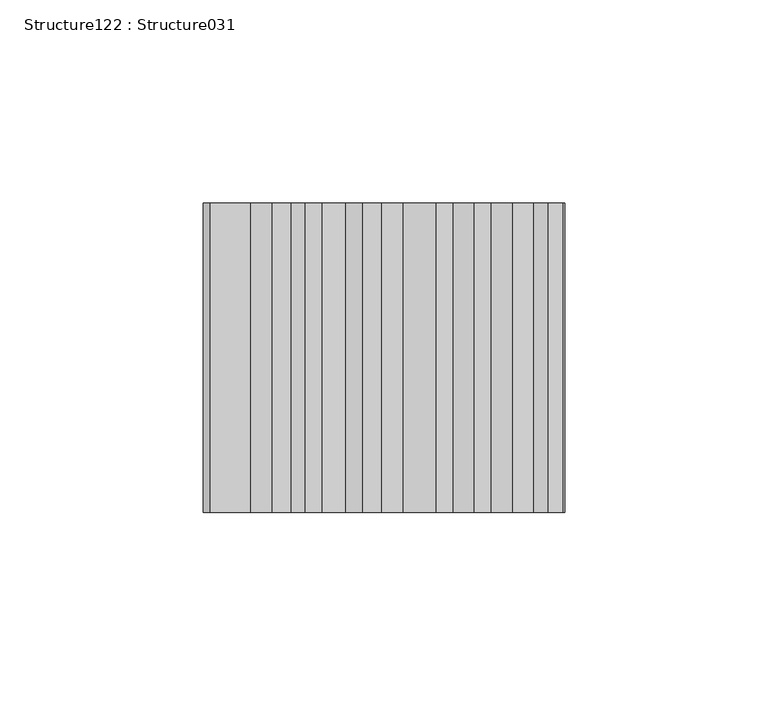
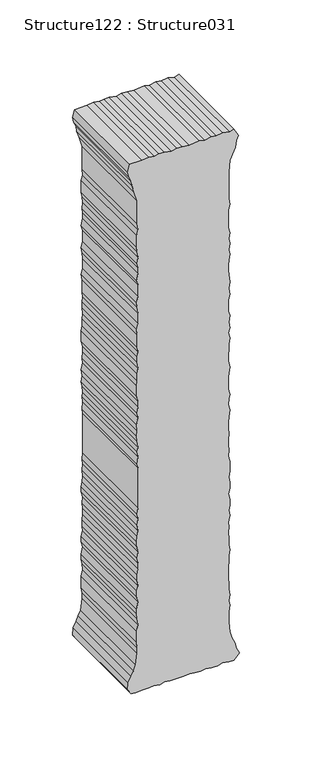
"""IFC4 building model written with IfcOpenShell, lengths in millimetres: proxy geometry, Structure122 : Structure031."""

from ifc_helpers import new_model, si_unit, frame, origin, place, context, project, spatial, polyline, outline, extrude, source, transform, mapped, element, save


def structure122_structure031_bc54f15f(model_context):
    return source(origin(), model_context, "Body", "SweptSolid", [
        extrude(outline(polyline([(3575.6853037, -45984.2637258), (3583.8864372, -45984.8461973), (3592.6700423, -45984.8461973), (3598.5284533, -45984.2637258), (3602.0280957, -45984.8461973), (3606.7295868, -45984.2637258), (3611.4134274, -45984.8461973), (3617.2718384, -45984.8461973), (3620.7971545, -45985.4382963), (3631.3410106, -45985.4382963), (3634.856699, -45984.8461973), (3640.114988, -45984.8461973), (3644.8245022, -45984.2637258), (3648.9258713, -45984.8461973), (3654.7842823, -45984.8461973), (3659.4584952, -45985.4382963), (3664.1423357, -45984.8461973), (3668.2437048, -45985.4382963), (3673.5276674, -45984.2637258), (3678.2018803, -45984.8461973), (3682.3289231, -45984.2637258), (3687.0127636, -45984.2637258), (3692.2710525, -45985.4382963), (3696.3884676, -45984.2637258), (3701.6547796, -45984.2637258), (3705.7545441, -45984.8461973), (3711.0304837, -45984.2637258), (3719.2316172, -45984.2637258), (3723.9154578, -45985.4382963), (3728.5992983, -45984.8461973), (3733.2991849, -45985.4382963), (3737.9750024, -45985.4382963), (3742.6748889, -45984.8461973), (3747.3587295, -45985.4382963), (3752.04257, -45985.4382963), (3756.7440611, -45984.8461973), (3762.5848215, -45984.2637258), (3767.2590344, -45985.4382963), (3771.9605256, -45984.8461973), (3775.4874463, -45984.2637258), (3780.1616592, -45985.4382963), (3790.7039107, -45985.4382963), (3798.9050443, -45984.2637258), (3804.1890069, -45985.4382963), (3808.8888934, -45985.4382963), (3813.5743386, -45984.8461973), (3817.6741031, -45984.8461973), (3822.932392, -45984.2637258), (3827.6162325, -45985.4382963), (3831.732043, -45984.2637258), (3836.4174882, -45984.8461973), (3842.2758992, -45984.2637258), (3845.8012153, -45985.4382963), (3855.7353217, -45985.4382963), (3859.8591552, -45984.2637258), (3865.1190488, -45984.8461973), (3870.4030114, -45984.2637258), (3879.7610648, -45985.4382963), (3884.4609514, -45985.4382963), (3888.5623205, -45984.8461973), (3893.246161, -45984.2637258), (3897.3475301, -45984.8461973), (3902.6314927, -45984.2637258), (3906.7328618, -45984.8461973), (3911.4054701, -45984.2637258), (3916.0909152, -45985.4382963), (3931.3346579, -45985.4382963), (3935.4328178, -45984.2637258), (3940.718385, -45984.8461973), (3962.9774586, -45984.8461973), (3972.3627903, -45984.2637258), (3981.7208437, -45979.5798853), (3987.5792547, -45978.9958093), (3991.0788971, -45977.2275351), (3997.5486624, -45980.7464328), (3996.390138, -45984.2637258), (3997.5486624, -45989.5396654), (3996.9645864, -45994.8059774), (3997.5486624, -45998.9153695), (3996.390138, -46004.1897044), (3997.5486624, -46008.2910735), (3996.390138, -46016.5002301), (3996.9645864, -46021.7665421), (3997.5486624, -46026.448778), (3996.390138, -46030.5501471), (3997.5486624, -46036.4085581), (3997.5486624, -46040.5099272), (3996.9645864, -46044.0272203), (3997.5486624, -46048.7206884), (3996.9645864, -46053.9950234), (3996.9645864, -46063.9531989), (3991.0788971, -46065.71345), (3986.4046842, -46064.5372749), (3982.3225704, -46062.7786284), (3978.2035506, -46062.1881339), (3972.3627903, -46060.4359058), (3964.1343784, -46058.0963925), (3944.8165449, -46058.0963925), (3939.5325823, -46057.5123164), (3935.4328178, -46058.6692363), (3925.4746423, -46058.6692363), (3921.3748778, -46058.0963925), (3916.6653636, -46057.5123164), (3911.4054701, -46058.0963925), (3907.888177, -46057.5123164), (3903.2059411, -46057.5123164), (3897.3475301, -46058.6692363), (3893.246161, -46057.5123164), (3883.8881076, -46057.5123164), (3878.5784713, -46058.6692363), (3874.5043805, -46058.0963925), (3869.2444869, -46057.5123164), (3861.0192843, -46057.5123164), (3856.3161885, -46058.6692363), (3851.6612309, -46058.0963925), (3841.0900965, -46058.0963925), (3836.9919366, -46057.5123164), (3832.8921721, -46058.0963925), (3828.2163546, -46058.0963925), (3822.932392, -46057.5123164), (3818.8310229, -46058.0963925), (3812.9726119, -46058.0963925), (3808.8888934, -46058.6692363), (3800.0876378, -46058.6692363), (3795.4037973, -46057.5123164), (3790.7039107, -46057.5123164), (3785.4456218, -46058.0963925), (3781.3282066, -46057.5123164), (3776.0618947, -46058.6692363), (3770.8036057, -46058.0963925), (3766.1021146, -46058.6692363), (3762.0023501, -46058.0963925), (3756.7440611, -46057.5123164), (3753.2171405, -46058.0963925), (3748.5429276, -46057.5123164), (3742.6748889, -46058.0963925), (3739.1592005, -46057.5123164), (3705.7545441, -46057.5123164), (3700.4705815, -46058.0963925), (3696.3884676, -46057.5123164), (3691.0868544, -46058.0963925), (3686.4030139, -46057.5123164), (3681.7271964, -46058.0963925), (3677.6274319, -46058.6692363), (3673.5276674, -46058.6692363), (3668.8261762, -46057.5123164), (3663.5598643, -46058.0963925), (3658.8840468, -46057.5123164), (3654.1841602, -46057.5123164), (3649.5003197, -46058.0963925), (3644.2420307, -46058.0963925), (3640.114988, -46057.5123164), (3636.0408972, -46058.6692363), (3631.3410106, -46058.6692363), (3626.6571701, -46057.5123164), (3620.7971545, -46058.6692363), (3616.69739, -46058.6692363), (3612.5976255, -46058.0963925), (3607.3393366, -46057.5123164), (3602.0280957, -46058.6692363), (3592.6700423, -46058.6692363), (3587.9685511, -46058.0963925), (3583.2863152, -46058.0963925), (3573.9266571, -46059.2613353), (3569.8268927, -46061.0199819), (3565.7094775, -46062.7786284), (3561.025637, -46065.129374), (3555.1848766, -46065.71345), (3551.0658569, -46062.7786284), (3550.4833855, -46059.2613353), (3551.0658569, -46054.5774948), (3551.0658569, -46048.7206884), (3551.6675836, -46045.2017908), (3550.4833855, -46039.9258512), (3551.6675836, -46036.4085581), (3551.0658569, -46031.7327406), (3551.0658569, -46021.174443), (3551.6675836, -46016.5002301), (3551.0658569, -46012.390838), (3550.4833855, -46007.6973699), (3551.0658569, -46003.5976054), (3550.4833855, -45998.9153695), (3550.4833855, -45993.6490575), (3551.6675836, -45990.1301599), (3550.4833855, -45984.8461973), (3550.4833855, -45980.7464328), (3555.1848766, -45976.6466683), (3559.8671125, -45978.9958093), (3565.1254015, -45980.1639613), (3569.8268927, -45982.5147069), (3575.6853037, -45984.2637258)])), frame((0.0, 247945.1599557, 0.0), z_axis=(0.0, 1.0, 0.0), x_axis=(0.0, 0.0, 1.0)), (0.0, 0.0, 1.0), 76.2),
    ])


if __name__ == "__main__":
    model = new_model("IFC4")
    model_context = context("Model", 3, world=origin())
    ifc_project = project(units=[si_unit("LENGTHUNIT", "METRE", prefix="MILLI")], contexts=[model_context])
    site = spatial("IfcSite", under=ifc_project)
    building = spatial("IfcBuilding", under=site)
    placement = place(None, origin())
    structure122_structure031_shape = structure122_structure031_bc54f15f(model_context)
    element("IfcBuildingElementProxy", 1, Name="Structure122 : Structure031", ObjectType="Structure122 : Structure031", at=placement, inside=building, context=model_context, shape_type="MappedRepresentation", body=[
        mapped(structure122_structure031_shape, transform((0.0, 0.0, 0.0), x_axis=(1.0, 0.0, 0.0), y_axis=(0.0, 1.0, 0.0), z_axis=(0.0, 0.0, 1.0))),
    ])
    save(model, "model.ifc")

# Revit data of these elements
# Type "Structure122 : Structure031"
#   NameOverride = "Structure031"
# Element 1 (IfcBuildingElementProxy, "Structure122 : Structure031")
#   Materials on its faces: "BRUSHED ALUM. LETTERING"
# Materials
#   "BRUSHED ALUM. LETTERING": class "Unassigned", colour RGB 169 181 186, transparency 0, Cost = 0
